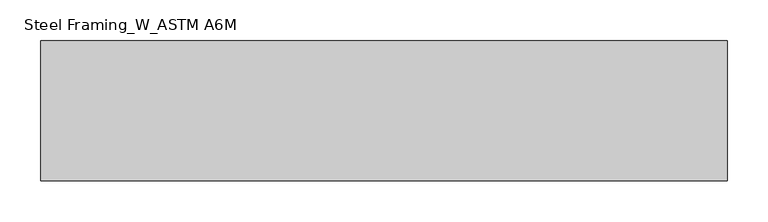
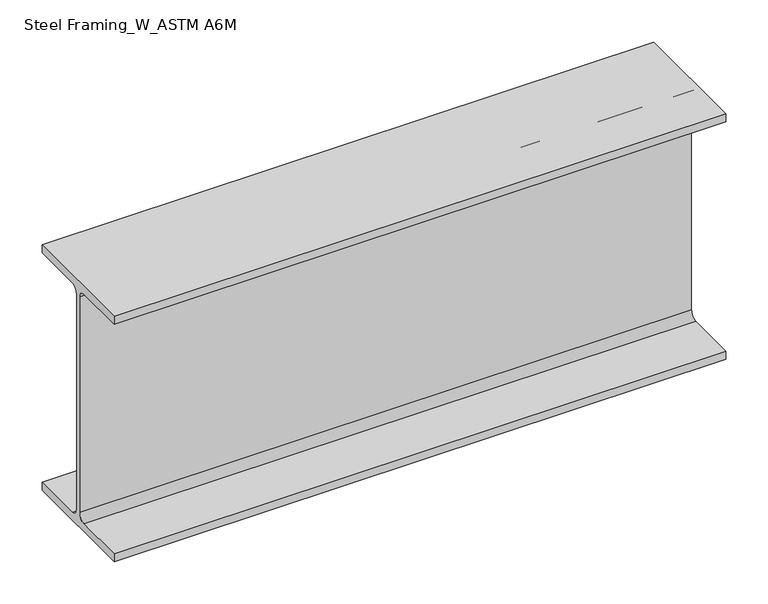
"""IFC4 building model written with IfcOpenShell, lengths in millimetres: beam geometry, Steel Framing_W_ASTM A6M : H_SB_AR_S02_W360x51_G3."""

from ifc_helpers import new_model, si_unit, point, frame, frame_2d, origin, place, context, project, spatial, polyline, circle_curve, trimmed, segment, composite_curve, outline, extrude, source, transform, mapped, element, save


def steel_framing_w_astm_a6m_0f62209b(model_context):
    return source(origin(), model_context, "Body", "SweptSolid", [
        extrude(outline(composite_curve([segment(polyline([(85.5, -166.4), (85.5, -178.0), (-85.5, -178.0), (-85.5, -166.4), (-13.72, -166.4)]), True, "CONTINUOUS"), segment(trimmed(circle_curve(frame_2d((-13.72, -156.3)), 10.1), [point((-13.72, -166.4))], [point((-3.62, -156.3))], True, "CARTESIAN"), True, "CONTINUOUS"), segment(polyline([(-3.62, -156.3), (-3.62, 156.3)]), True, "CONTINUOUS"), segment(trimmed(circle_curve(frame_2d((-13.72, 156.3)), 10.1), [point((-3.62, 156.3))], [point((-13.72, 166.4))], True, "CARTESIAN"), True, "CONTINUOUS"), segment(polyline([(-13.72, 166.4), (-85.5, 166.4), (-85.5, 178.0), (85.5, 178.0), (85.5, 166.4), (13.72, 166.4)]), True, "CONTINUOUS"), segment(trimmed(circle_curve(frame_2d((13.72, 156.3)), 10.1), [point((13.72, 166.4))], [point((3.62, 156.3))], True, "CARTESIAN"), True, "CONTINUOUS"), segment(polyline([(3.62, 156.3), (3.62, -156.3)]), True, "CONTINUOUS"), segment(trimmed(circle_curve(frame_2d((13.72, -156.3)), 10.1), [point((3.62, -156.3))], [point((13.72, -166.4))], True, "CARTESIAN"), True, "CONTINUOUS"), segment(polyline([(13.72, -166.4), (85.5, -166.4)]), True, "CONTINUOUS")], self_intersect=False)), frame((-253.8, 0.0, 0.0), z_axis=(1.0, 0.0, 0.0), x_axis=(0.0, 1.0, 0.0)), (0.0, 0.0, 1.0), 839.3),
    ])


if __name__ == "__main__":
    model = new_model("IFC4")
    model_context = context("Model", 3, world=origin())
    ifc_project = project(units=[si_unit("LENGTHUNIT", "METRE", prefix="MILLI")], contexts=[model_context])
    site = spatial("IfcSite", under=ifc_project)
    building = spatial("IfcBuilding", under=site)
    placement = place(None, origin())
    steel_framing_w_astm_a6m_shape = steel_framing_w_astm_a6m_0f62209b(model_context)
    element("IfcBeam", 1, ObjectType="Steel Framing_W_ASTM A6M : H_SB_AR_S02_W360x51_G3", at=placement, inside=building, context=model_context, shape_type="MappedRepresentation", body=[
        mapped(steel_framing_w_astm_a6m_shape, transform((0.0, 0.0, 0.0), x_axis=(1.0, 0.0, 0.0), y_axis=(0.0, 1.0, 0.0), z_axis=(0.0, 0.0, 1.0))),
    ])
    save(model, "model.ifc")

# Revit data of these elements
# Type "Steel Framing_W_ASTM A6M : H_SB_AR_S02_W360x51_G3"
#   Type Mark = "G3"
#   Section Name Key = "W14x34"
#   Width = 17.1 cm
#   Web Thickness = 0.724 cm
#   Web Fillet = 1.01 cm
#   Warping Constant = 287000.0 cm⁶
#   Torsional Moment of Inertia = 23.70 cm⁴
#   Section Area = 64.5 cm²
#   Plastic Modulus weak axis = 174.0 cm³
#   Plastic Modulus strong axis = 895.0 cm³
#   Perimeter = 1.36 m²/m
#   Nominal Weight = 51.00 kgf/m
#   Moment of Inertia weak axis = 970.00 cm⁴
#   Moment of Inertia strong axis = 14200.00 cm⁴
#   Height = 35.6 cm
#   Flange Thickness = 1.16 cm
#   Elastic Modulus weak axis = 113.0 cm³
#   Elastic Modulus strong axis = 796.0 cm³
#   Centroid Vertical = 17.8 cm
#   Centroid Horizontal = 8.55 cm
#   Length [instance default] = 1500 mm
#   Structural Material [instance default] = Steel, 45-345
#   Bolt Spacing = 0
#   Assembly Code = ""
# Element 1 (IfcBeam, "Steel Framing_W_ASTM A6M : H_SB_AR_S02_W360x51_G3")
#   Materials on its faces: "Steel, 45-345"
# Materials
#   "Steel, 45-345": class "Metal", colour RGB 189 187 185, transparency 0, Description = "Steel 345 MPa", Cost = 0
